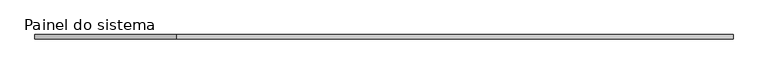
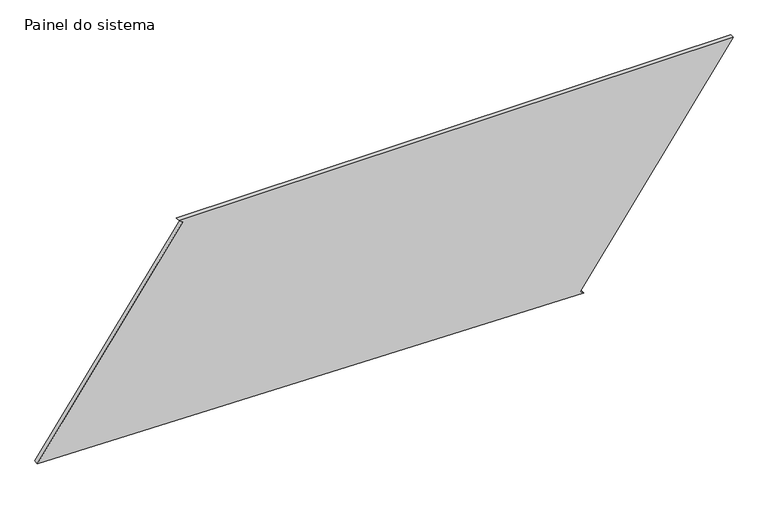
"""IFC4 building model written with IfcOpenShell, lengths in millimetres: plate geometry, Painel do sistema : Envidraçado."""

from ifc_helpers import new_model, si_unit, frame, origin, place, context, project, spatial, polyline, outline, extrude, source, transform, mapped, element, save


def painel_do_sistema_a7b7bcb7(model_context):
    return source(origin(), model_context, "Body", "SweptSolid", [
        extrude(outline(polyline([(0.0, 1119.7697081), (14.4529738, 1099.3708957), (1229.0658516, 1959.9488426), (1229.0658516, -1162.3272069), (1214.6128778, -1141.9283945), (60.0653158, -1959.9488426), (0.0, 1119.7697081)])), frame((0.0, 24.5, 0.0), z_axis=(0.0, 1.0, 0.0), x_axis=(0.0, 0.0, 1.0)), (0.0, 0.0, 1.0), 25.0),
    ])


if __name__ == "__main__":
    model = new_model("IFC4")
    model_context = context("Model", 3, world=origin())
    ifc_project = project(units=[si_unit("LENGTHUNIT", "METRE", prefix="MILLI")], contexts=[model_context])
    site = spatial("IfcSite", under=ifc_project)
    building = spatial("IfcBuilding", under=site)
    placement = place(None, origin())
    painel_do_sistema_shape = painel_do_sistema_a7b7bcb7(model_context)
    element("IfcPlate", 1, ObjectType="Painel do sistema : Envidraçado", at=placement, inside=building, context=model_context, shape_type="MappedRepresentation", body=[
        mapped(painel_do_sistema_shape, transform((0.0, 0.0, 0.0), x_axis=(1.0, 0.0, 0.0), y_axis=(0.0, 1.0, 0.0), z_axis=(0.0, 0.0, 1.0))),
    ])
    save(model, "model.ifc")

# Revit data of these elements
# Type "Painel do sistema : Envidraçado"
#   Construction Type Id = "GSP4R"
#   Analytic Construction = "Vidraça única Pilkington 1/8 pol"
#   Visual Light Transmittance = 0.9
#   Solar Heat Gain Coefficient = 0.86
#   Heat Transfer Coefficient (U) = 6.7069 W/(m²·K)
# Element 1 (IfcPlate, "Painel do sistema : Envidraçado")
#   Materials on its faces: "Vidro"
# Materials
#   "Vidro": class "Vidro", colour RGB 0 128 192, transparency 0.9, Description = "Vidro de sílica", Cost = 0
